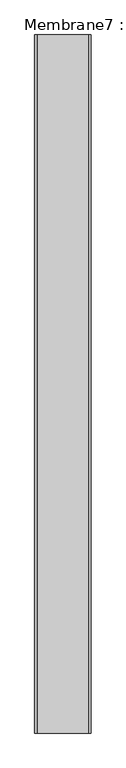
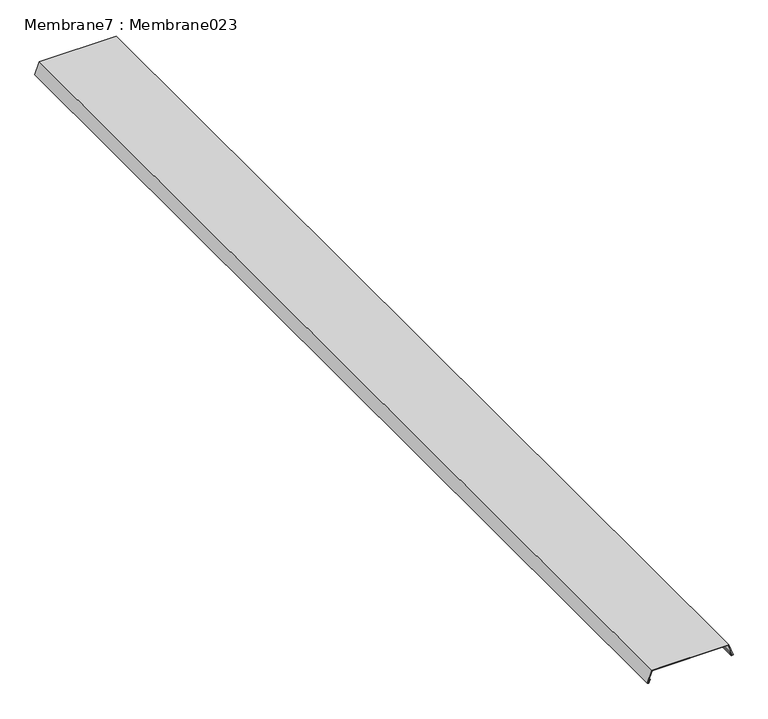
"""IFC4 building model written with IfcOpenShell, lengths in millimetres: proxy geometry, Membrane7 : Membrane023."""

from ifc_helpers import new_model, si_unit, frame, origin, place, context, project, spatial, polyline, outline, extrude, source, transform, mapped, element, save


def membrane7_membrane023_d6f66529(model_context):
    return source(origin(), model_context, "Body", "SweptSolid", [
        extrude(outline(polyline([(40168.6784303, -7256.3081811), (40145.4975649, -7264.7453261), (40144.2932564, -7261.4365157), (40151.4620885, -7258.8272742), (40151.8041086, -7259.7669668), (40145.5749692, -7262.0341881), (40146.0952374, -7263.4636133), (40167.6784303, -7255.6079735), (40167.6784303, -7111.8130831), (40146.0952374, -7103.9574433), (40145.5749692, -7105.3868685), (40151.8041086, -7107.6540898), (40151.4620885, -7108.5937825), (40144.2932564, -7105.984541), (40145.4975649, -7102.6757306), (40168.6784303, -7111.1128756), (40168.6784303, -7256.3081811)])), frame((0.0, 7182.1531721, 0.0), z_axis=(0.0, 1.0, 0.0), x_axis=(0.0, 0.0, 1.0)), (0.0, 0.0, 1.0), 2000.0),
    ])


if __name__ == "__main__":
    model = new_model("IFC4")
    model_context = context("Model", 3, world=origin())
    ifc_project = project(units=[si_unit("LENGTHUNIT", "METRE", prefix="MILLI")], contexts=[model_context])
    site = spatial("IfcSite", under=ifc_project)
    building = spatial("IfcBuilding", under=site)
    placement = place(None, origin())
    membrane7_membrane023_shape = membrane7_membrane023_d6f66529(model_context)
    element("IfcBuildingElementProxy", 1, Name="Membrane7 : Membrane023", ObjectType="Membrane7 : Membrane023", at=placement, inside=building, context=model_context, shape_type="MappedRepresentation", body=[
        mapped(membrane7_membrane023_shape, transform((0.0, 0.0, 0.0), x_axis=(1.0, 0.0, 0.0), y_axis=(0.0, 1.0, 0.0), z_axis=(0.0, 0.0, 1.0))),
    ])
    save(model, "model.ifc")

# Revit data of these elements
# Type "Membrane7 : Membrane023"
#   NameOverride = "Membrane023"
# Element 1 (IfcBuildingElementProxy, "Membrane7 : Membrane023")
#   Materials on its faces: "16 GA. COPPER FLASHING"
# Materials
#   "16 GA. COPPER FLASHING": class "Unassigned", colour RGB 251 232 155, transparency 0, Cost = 0
